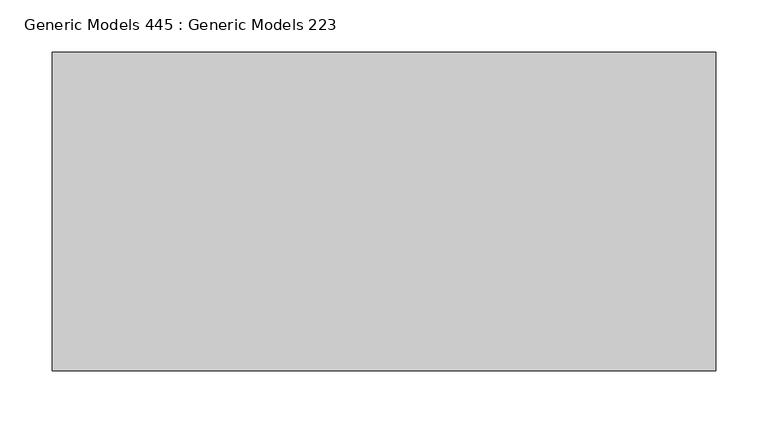
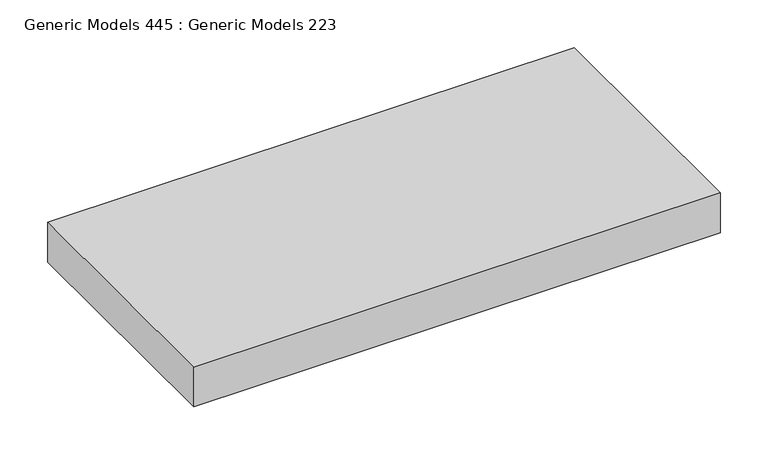
"""IFC4 building model written with IfcOpenShell, lengths in millimetres: proxy geometry, Generic Models 445 : Generic Models 223."""

import ifcopenshell
import ifcopenshell.guid

model = None  # the IFC model being written
_history = None  # IfcOwnerHistory: only IFC2X3 demands one
_inside = {}  # id of a spatial element -> (the spatial element, [elements in it])
_under = {}  # id of a project, library or spatial element -> (it, [spatial elements below it])
_declared = {}  # id of a project -> (the project, [libraries it declares])
_typed = {}  # id of a type object -> (the type object, [elements of that type])
_made_of = {}  # id of a material, layer set ... -> (it, [elements and type objects made of it])


def new_model(schema):
    """Start an empty IFC model of exactly this schema.

    Asked for "IFC4X3", IfcOpenShell would pick the latest addendum, in which some entities
    have other attributes; the version numbers below select the first issue.
    IFC2X3 requires an IfcOwnerHistory on every rooted entity: one is made here for all.
    """
    global model, _history
    if schema == "IFC4X3":
        model = ifcopenshell.file(schema_version=(4, 3, 0, 0))
    else:
        model = ifcopenshell.file(schema=schema)
    _inside.clear()
    _under.clear()
    _declared.clear()
    _typed.clear()
    _made_of.clear()
    _history = None
    if model.schema == "IFC2X3":
        org = make("IfcOrganization", Name="unknown")
        user = make(
            "IfcPersonAndOrganization",
            ThePerson=make("IfcPerson", FamilyName="unknown"),
            TheOrganization=org,
        )
        app = make(
            "IfcApplication",
            ApplicationDeveloper=org,
            Version="unknown",
            ApplicationFullName="unknown",
            ApplicationIdentifier="unknown",
        )
        _history = make(
            "IfcOwnerHistory",
            OwningUser=user,
            OwningApplication=app,
            ChangeAction="ADDED",
            CreationDate=0,
        )
    return model


def make(cls, **values):
    """One entity of the class cls with the attributes given. An attribute that is None is left unset."""
    return model.create_entity(
        cls, **{name: value for name, value in values.items() if value is not None}
    )


def rooted(cls, **values):
    """An entity with a GlobalId (a new one), such as an element, a storey or a relation."""
    return make(cls, GlobalId=ifcopenshell.guid.new(), OwnerHistory=_history, **values)


def si_unit(unit_type, name, prefix=None):
    """IfcSIUnit, for example si_unit("LENGTHUNIT", "METRE", prefix="MILLI")."""
    return make("IfcSIUnit", UnitType=unit_type, Prefix=prefix, Name=name)


def assignment(units):
    """IfcUnitAssignment: the units of a project."""
    return None if units is None else make("IfcUnitAssignment", Units=units)


def point(xyz):
    """IfcCartesianPoint."""
    return None if xyz is None else make("IfcCartesianPoint", Coordinates=xyz)


def direction(xyz):
    """IfcDirection."""
    return None if xyz is None else make("IfcDirection", DirectionRatios=xyz)


def frame(location, z_axis=None, x_axis=None):
    """IfcAxis2Placement3D, a coordinate frame: its origin and axes. An axis left out is left unset."""
    return make(
        "IfcAxis2Placement3D",
        Location=point(location),
        Axis=direction(z_axis),
        RefDirection=direction(x_axis),
    )


def origin():
    """The frame at (0, 0, 0) with its axes left unset."""
    return frame((0.0, 0.0, 0.0))


def place(relative_to, where):
    """IfcLocalPlacement: puts the frame where relative to a parent placement (None: the world)."""
    return make(
        "IfcLocalPlacement", PlacementRelTo=relative_to, RelativePlacement=where
    )


def context(
    kind, dimensions, precision=None, world=None, true_north=None, identifier=None
):
    """IfcGeometricRepresentationContext, for example the 3D "Model" context."""
    return make(
        "IfcGeometricRepresentationContext",
        ContextIdentifier=identifier,
        ContextType=kind,
        CoordinateSpaceDimension=dimensions,
        Precision=precision,
        WorldCoordinateSystem=world,
        TrueNorth=true_north,
    )


def project(units=None, contexts=None):
    """IfcProject with its units and contexts."""
    return rooted(
        "IfcProject",
        Name="project",
        RepresentationContexts=contexts,
        UnitsInContext=assignment(units),
    )


def spatial(cls, under=None, at=None, **own):
    """A site, building, storey or space (cls), placed at a placement, below another one or the project."""
    s = rooted(cls, ObjectPlacement=at, **own)
    if under is not None:
        _under.setdefault(under.id(), (under, []))[1].append(s)
    return s


def polyline(points):
    """IfcPolyline through the points."""
    return make("IfcPolyline", Points=[point(p) for p in points])


def outline(outer, holes=None, kind="AREA"):
    """IfcArbitraryClosedProfileDef: a profile drawn as a closed curve; with holes, ...WithVoids."""
    if holes is None:
        return make("IfcArbitraryClosedProfileDef", ProfileType=kind, OuterCurve=outer)
    return make(
        "IfcArbitraryProfileDefWithVoids",
        ProfileType=kind,
        OuterCurve=outer,
        InnerCurves=holes,
    )


def extrude(swept, where, along, depth):
    """IfcExtrudedAreaSolid: the profile swept, set in the frame where, extruded along a direction by depth."""
    return make(
        "IfcExtrudedAreaSolid",
        SweptArea=swept,
        Position=where,
        ExtrudedDirection=direction(along),
        Depth=depth,
    )


def shape(context_of_items, identifier, shape_type, items):
    """IfcShapeRepresentation: the items that make up one representation, for example the "Body"."""
    return make(
        "IfcShapeRepresentation",
        ContextOfItems=context_of_items,
        RepresentationIdentifier=identifier,
        RepresentationType=shape_type,
        Items=items,
    )


def source(mapping_origin, context_of_items, identifier, shape_type, items):
    """IfcRepresentationMap: a shape defined once, which mapped items show again and again."""
    return make(
        "IfcRepresentationMap",
        MappingOrigin=mapping_origin,
        MappedRepresentation=shape(context_of_items, identifier, shape_type, items),
    )


def transform(
    local_origin,
    x_axis=None,
    y_axis=None,
    z_axis=None,
    scale=None,
    scale2=None,
    scale3=None,
    uniform=True,
):
    """IfcCartesianTransformationOperator3D, or its non-uniform kind. x_axis, y_axis, z_axis: its Axis1, 2, 3."""
    if uniform:
        return make(
            "IfcCartesianTransformationOperator3D",
            Axis1=direction(x_axis),
            Axis2=direction(y_axis),
            LocalOrigin=point(local_origin),
            Scale=scale,
            Axis3=direction(z_axis),
        )
    return make(
        "IfcCartesianTransformationOperator3DnonUniform",
        Axis1=direction(x_axis),
        Axis2=direction(y_axis),
        LocalOrigin=point(local_origin),
        Scale=scale,
        Axis3=direction(z_axis),
        Scale2=scale2,
        Scale3=scale3,
    )


def mapped(mapping_source, mapping_target):
    """IfcMappedItem: shows the shape of a source again, moved by a transform."""
    return make(
        "IfcMappedItem", MappingSource=mapping_source, MappingTarget=mapping_target
    )


def made_of(thing, what):
    """Note that an element or type object is made of a material, layer set ...; save() writes the relation."""
    if what is not None:
        _made_of.setdefault(what.id(), (what, []))[1].append(thing)
    return thing


def element(
    cls,
    number,
    at=None,
    inside=None,
    cuts=None,
    type_object=None,
    material=None,
    context=None,
    identifier="Body",
    shape_type=None,
    held_by="IfcProductDefinitionShape",
    body=None,
    shapes=None,
    **own,
):
    """One element of the class cls, such as IfcWall. Its Tag is "e" and its number.

    at: its placement. inside: the storey or other place that contains it. cuts: it is an
    opening in that element (IfcRelVoidsElement). A single representation is given by context,
    identifier, shape_type and body (its items); several are given by shapes. held_by: the class
    of the entity that holds the representations. save() writes the other relations.
    """
    e = rooted(cls, Tag="e%d" % number, ObjectPlacement=at, **own)
    if body is not None:
        shapes = [shape(context, identifier, shape_type, body)]
    if shapes is not None:
        e.Representation = make(held_by, Representations=shapes)
    if inside is not None:
        _inside.setdefault(inside.id(), (inside, []))[1].append(e)
    if cuts is not None:
        rooted(
            "IfcRelVoidsElement", RelatingBuildingElement=cuts, RelatedOpeningElement=e
        )
    if type_object is not None:
        _typed.setdefault(type_object.id(), (type_object, []))[1].append(e)
    return made_of(e, material)


def aggregate(whole, parts):
    """IfcRelAggregates: a whole, such as a stair, and the parts it consists of."""
    return rooted("IfcRelAggregates", RelatingObject=whole, RelatedObjects=parts)


def save(model, path):
    """Write the relations noted so far, then the file.

    IfcRelAggregates (storeys below a building ...), IfcRelContainedInSpatialStructure (elements
    in a storey), IfcRelDefinesByType, IfcRelAssociatesMaterial and IfcRelDeclares: one each for
    every whole, place, type object, material and project.
    """
    for whole, parts in _under.values():
        aggregate(whole, parts)
    for where, things in _inside.values():
        rooted(
            "IfcRelContainedInSpatialStructure",
            RelatedElements=things,
            RelatingStructure=where,
        )
    for kind, things in _typed.values():
        rooted("IfcRelDefinesByType", RelatedObjects=things, RelatingType=kind)
    for what, things in _made_of.values():
        rooted("IfcRelAssociatesMaterial", RelatedObjects=things, RelatingMaterial=what)
    for by, libraries in _declared.values():
        rooted("IfcRelDeclares", RelatingContext=by, RelatedDefinitions=libraries)
    model.write(path)


def generic_models_445_generic_models_223_24cea836(model_context):
    return source(origin(), model_context, "Body", "SweptSolid", [
        extrude(outline(polyline([(7556.3263704, 4564.8872686), (8191.3263705, 4564.8872686), (8191.3263705, 4260.0872686), (7556.3263704, 4260.0872686), (7556.3263704, 4564.8872686)])), frame((0.0, 0.0, 123500.896), z_axis=(0.0, 0.0, 1.0), x_axis=(1.0, 0.0, 0.0)), (0.0, 0.0, 1.0), 50.8),
    ])


if __name__ == "__main__":
    model = new_model("IFC4")
    model_context = context("Model", 3, world=origin())
    ifc_project = project(units=[si_unit("LENGTHUNIT", "METRE", prefix="MILLI")], contexts=[model_context])
    site = spatial("IfcSite", under=ifc_project)
    building = spatial("IfcBuilding", under=site)
    placement = place(None, origin())
    generic_models_445_generic_models_223_shape = generic_models_445_generic_models_223_24cea836(model_context)
    element("IfcBuildingElementProxy", 1, Name="Generic Models 445 : Generic Models 223", ObjectType="Generic Models 445 : Generic Models 223", at=placement, inside=building, context=model_context, shape_type="MappedRepresentation", body=[
        mapped(generic_models_445_generic_models_223_shape, transform((0.0, 0.0, 0.0), x_axis=(1.0, 0.0, 0.0), y_axis=(0.0, 1.0, 0.0), z_axis=(0.0, 0.0, 1.0))),
    ])
    save(model, "model.ifc")

# Revit data of these elements
# Element 1 (IfcBuildingElementProxy, "Generic Models 445 : Generic Models 223")
#   Materials on its faces: "_2\" SAND"
# Materials
#   "_2\" SAND": class "Generic", colour RGB 245 226 173, transparency 0, Cost = 0
